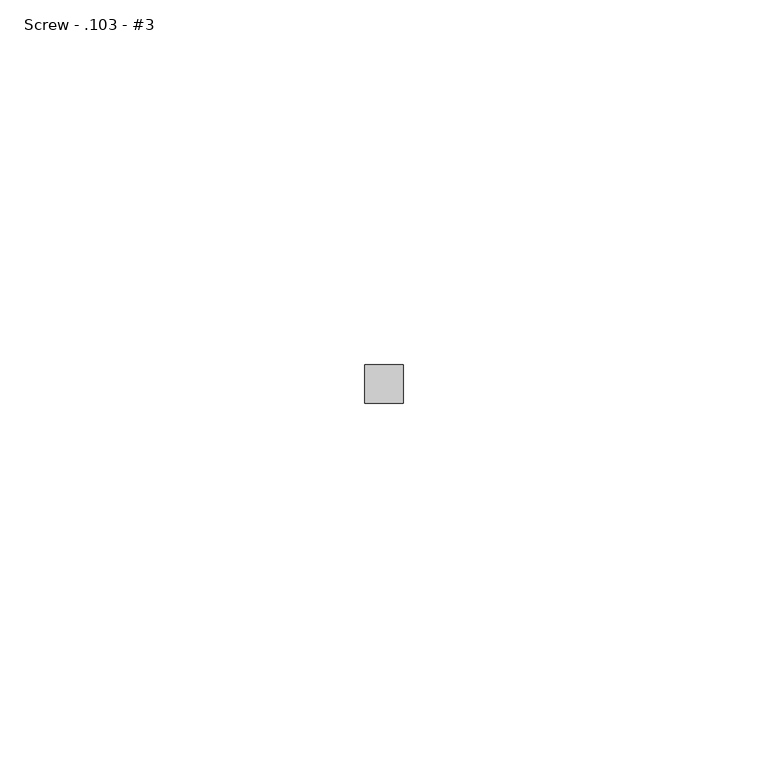
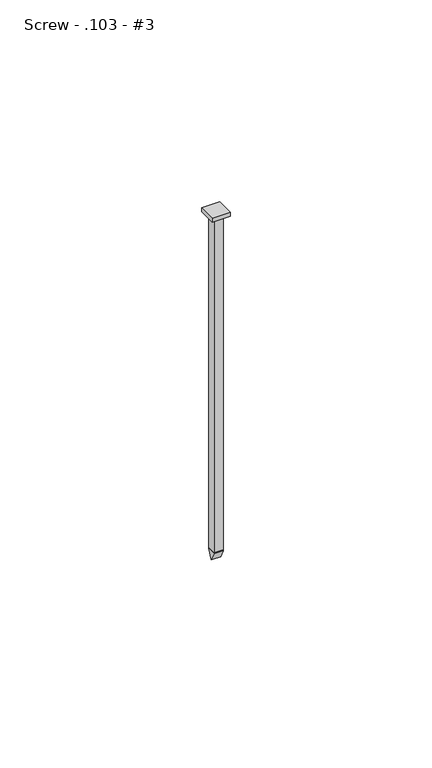
"""IFC4 building model written with IfcOpenShell, lengths in millimetres: fastener geometry, 060523 - W_P_C - Fastenings - Generic - SQUARE : Screw - .103 - #3."""

from ifc_helpers import new_model, si_unit, frame, origin, origin_with_axes, place, context, project, spatial, polyline, outline, extrude, source, transform, mapped, element, save


def screw_103_3_3ef0f881(model_context):
    return source(origin(), model_context, "Body", "SweptSolid", [
        extrude(outline(polyline([(0.0, -104.2162), (-1.3081, -101.6), (1.3081, -101.6), (0.0, -104.2162)])), frame((-1.3081, 0.0, 0.0), z_axis=(1.0, 0.0, 0.0), x_axis=(0.0, 1.0, 0.0)), (0.0, 0.0, 1.0), 2.6162),
        extrude(outline(polyline([(-2.6162, -2.6162), (-2.6162, 2.6162), (2.6162, 2.6162), (2.6162, -2.6162), (-2.6162, -2.6162)])), origin_with_axes(), (0.0, 0.0, 1.0), 1.3081),
        extrude(outline(polyline([(-1.3081, 1.3081), (1.3081, 1.3081), (1.3081, -1.3081), (-1.3081, -1.3081), (-1.3081, 1.3081)])), frame((0.0, 0.0, -101.6), z_axis=(0.0, 0.0, 1.0), x_axis=(1.0, 0.0, 0.0)), (0.0, 0.0, 1.0), 101.6),
    ])


if __name__ == "__main__":
    model = new_model("IFC4")
    model_context = context("Model", 3, world=origin())
    ifc_project = project(units=[si_unit("LENGTHUNIT", "METRE", prefix="MILLI")], contexts=[model_context])
    site = spatial("IfcSite", under=ifc_project)
    building = spatial("IfcBuilding", under=site)
    placement = place(None, origin())
    screw_103_3_shape = screw_103_3_3ef0f881(model_context)
    element("IfcFastener", 1, ObjectType="060523 - W_P_C - Fastenings - Generic - SQUARE : Screw - .103 - #3", at=placement, inside=building, context=model_context, shape_type="MappedRepresentation", body=[
        mapped(screw_103_3_shape, transform((0.0, 0.0, 0.0), x_axis=(1.0, 0.0, 0.0), y_axis=(0.0, 1.0, 0.0), z_axis=(0.0, 0.0, 1.0))),
    ])
    save(model, "model.ifc")

# Revit data of these elements
# Type "060523 - W_P_C - Fastenings - Generic - SQUARE : Screw - .103 - #3"
#   Washer_Thickness = 0' - 0.00333"
#   Washer Radius = 0' - 0.0615"
#   Washer Offset - Head = 0' - 0"
#   Washer Offset = 0' - 0"
#   Thickness_of_Substrate [instance default] = 0' - 1"
#   Side = 0' - 0 37/64"
#   Radius = 0' - 0.0515"
#   Length [instance default] = 0' - 4"
#   Head Size = 0' - 1"
#   Head Radius = 0' - 0 1/2"
#   Head Height = 0' - 0.01"
#   Double Diameter = 0' - 0.206"
#   Diameter = 0' - 0.103"
#   Default Elevation = 4' - 0"
#   Washer_Nut_Visibility = no
#   Washer_Head_Visibility = no
#   Round_Head_Visibility = yes
#   Point Visibility = yes
#   Nut_Visibility = no
#   Hex_Head_Visiblilty = no
#   Washer Material = none
#   Bolt Material (Size) = AT SILL - FASTENER AT 24" O.C.
# Materials
#   "AT SILL - FASTENER AT 24\" O.C.": class "Generic", colour RGB 120 120 120, transparency 0, Cost = 0
